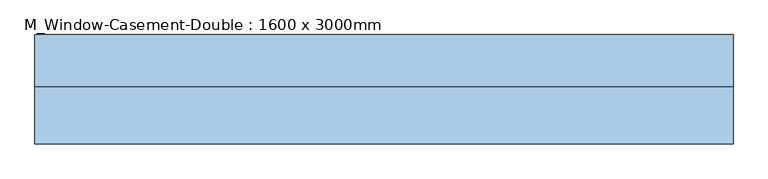
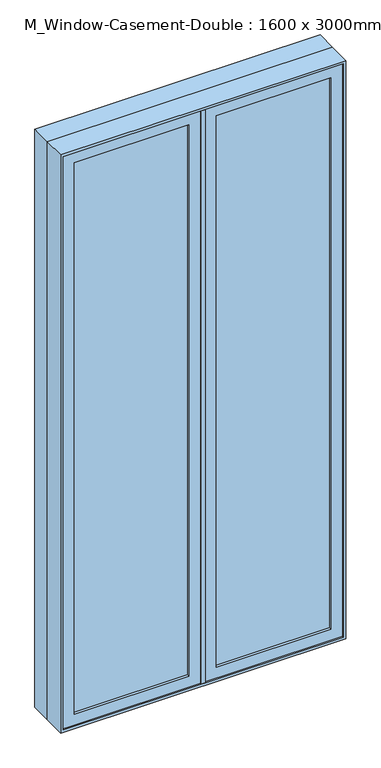
"""IFC4 building model written with IfcOpenShell, lengths in millimetres: window geometry, M_Window-Casement-Double : 1600 x 3000mm."""

import ifcopenshell
import ifcopenshell.guid

model = None  # the IFC model being written
_history = None  # IfcOwnerHistory: only IFC2X3 demands one
_inside = {}  # id of a spatial element -> (the spatial element, [elements in it])
_under = {}  # id of a project, library or spatial element -> (it, [spatial elements below it])
_declared = {}  # id of a project -> (the project, [libraries it declares])
_typed = {}  # id of a type object -> (the type object, [elements of that type])
_made_of = {}  # id of a material, layer set ... -> (it, [elements and type objects made of it])


def new_model(schema):
    """Start an empty IFC model of exactly this schema.

    Asked for "IFC4X3", IfcOpenShell would pick the latest addendum, in which some entities
    have other attributes; the version numbers below select the first issue.
    IFC2X3 requires an IfcOwnerHistory on every rooted entity: one is made here for all.
    """
    global model, _history
    if schema == "IFC4X3":
        model = ifcopenshell.file(schema_version=(4, 3, 0, 0))
    else:
        model = ifcopenshell.file(schema=schema)
    _inside.clear()
    _under.clear()
    _declared.clear()
    _typed.clear()
    _made_of.clear()
    _history = None
    if model.schema == "IFC2X3":
        org = make("IfcOrganization", Name="unknown")
        user = make(
            "IfcPersonAndOrganization",
            ThePerson=make("IfcPerson", FamilyName="unknown"),
            TheOrganization=org,
        )
        app = make(
            "IfcApplication",
            ApplicationDeveloper=org,
            Version="unknown",
            ApplicationFullName="unknown",
            ApplicationIdentifier="unknown",
        )
        _history = make(
            "IfcOwnerHistory",
            OwningUser=user,
            OwningApplication=app,
            ChangeAction="ADDED",
            CreationDate=0,
        )
    return model


def make(cls, **values):
    """One entity of the class cls with the attributes given. An attribute that is None is left unset."""
    return model.create_entity(
        cls, **{name: value for name, value in values.items() if value is not None}
    )


def rooted(cls, **values):
    """An entity with a GlobalId (a new one), such as an element, a storey or a relation."""
    return make(cls, GlobalId=ifcopenshell.guid.new(), OwnerHistory=_history, **values)


def si_unit(unit_type, name, prefix=None):
    """IfcSIUnit, for example si_unit("LENGTHUNIT", "METRE", prefix="MILLI")."""
    return make("IfcSIUnit", UnitType=unit_type, Prefix=prefix, Name=name)


def assignment(units):
    """IfcUnitAssignment: the units of a project."""
    return None if units is None else make("IfcUnitAssignment", Units=units)


def point(xyz):
    """IfcCartesianPoint."""
    return None if xyz is None else make("IfcCartesianPoint", Coordinates=xyz)


def direction(xyz):
    """IfcDirection."""
    return None if xyz is None else make("IfcDirection", DirectionRatios=xyz)


def frame(location, z_axis=None, x_axis=None):
    """IfcAxis2Placement3D, a coordinate frame: its origin and axes. An axis left out is left unset."""
    return make(
        "IfcAxis2Placement3D",
        Location=point(location),
        Axis=direction(z_axis),
        RefDirection=direction(x_axis),
    )


def origin():
    """The frame at (0, 0, 0) with its axes left unset."""
    return frame((0.0, 0.0, 0.0))


def place(relative_to, where):
    """IfcLocalPlacement: puts the frame where relative to a parent placement (None: the world)."""
    return make(
        "IfcLocalPlacement", PlacementRelTo=relative_to, RelativePlacement=where
    )


def context(
    kind, dimensions, precision=None, world=None, true_north=None, identifier=None
):
    """IfcGeometricRepresentationContext, for example the 3D "Model" context."""
    return make(
        "IfcGeometricRepresentationContext",
        ContextIdentifier=identifier,
        ContextType=kind,
        CoordinateSpaceDimension=dimensions,
        Precision=precision,
        WorldCoordinateSystem=world,
        TrueNorth=true_north,
    )


def project(units=None, contexts=None):
    """IfcProject with its units and contexts."""
    return rooted(
        "IfcProject",
        Name="project",
        RepresentationContexts=contexts,
        UnitsInContext=assignment(units),
    )


def spatial(cls, under=None, at=None, **own):
    """A site, building, storey or space (cls), placed at a placement, below another one or the project."""
    s = rooted(cls, ObjectPlacement=at, **own)
    if under is not None:
        _under.setdefault(under.id(), (under, []))[1].append(s)
    return s


def polyline(points):
    """IfcPolyline through the points."""
    return make("IfcPolyline", Points=[point(p) for p in points])


def outline(outer, holes=None, kind="AREA"):
    """IfcArbitraryClosedProfileDef: a profile drawn as a closed curve; with holes, ...WithVoids."""
    if holes is None:
        return make("IfcArbitraryClosedProfileDef", ProfileType=kind, OuterCurve=outer)
    return make(
        "IfcArbitraryProfileDefWithVoids",
        ProfileType=kind,
        OuterCurve=outer,
        InnerCurves=holes,
    )


def extrude(swept, where, along, depth):
    """IfcExtrudedAreaSolid: the profile swept, set in the frame where, extruded along a direction by depth."""
    return make(
        "IfcExtrudedAreaSolid",
        SweptArea=swept,
        Position=where,
        ExtrudedDirection=direction(along),
        Depth=depth,
    )


def faces_of(points, faces, orient=None, outer=None):
    """IfcFace entities. A face is a list of loops; a loop is a list of indices into points, from 0.

    orient and outer hold one flag for each loop. By default every Orientation is true, the
    first loop of a face is its IfcFaceOuterBound and the others are IfcFaceBound.
    """
    made = []
    for i, loops in enumerate(faces):
        bounds = []
        for j, loop in enumerate(loops):
            is_outer = j == 0 if outer is None else outer[i][j]
            bounds.append(
                make(
                    "IfcFaceOuterBound" if is_outer else "IfcFaceBound",
                    Bound=make("IfcPolyLoop", Polygon=[points[k] for k in loop]),
                    Orientation=True if orient is None else orient[i][j],
                )
            )
        made.append(make("IfcFace", Bounds=bounds))
    return made


def faceted_brep(points, faces, orient=None, outer=None, voids=None):
    """IfcFacetedBrep: a solid bounded by flat faces; with voids (closed shells), ...WithVoids."""
    shared = [point(p) for p in points]
    hull = make("IfcClosedShell", CfsFaces=faces_of(shared, faces, orient, outer))
    if voids is None:
        return make("IfcFacetedBrep", Outer=hull)
    return make(
        "IfcFacetedBrepWithVoids",
        Outer=hull,
        Voids=[
            make(cls, CfsFaces=faces_of(shared, fs, o, b)) for cls, fs, o, b in voids
        ],
    )


def shape(context_of_items, identifier, shape_type, items):
    """IfcShapeRepresentation: the items that make up one representation, for example the "Body"."""
    return make(
        "IfcShapeRepresentation",
        ContextOfItems=context_of_items,
        RepresentationIdentifier=identifier,
        RepresentationType=shape_type,
        Items=items,
    )


def source(mapping_origin, context_of_items, identifier, shape_type, items):
    """IfcRepresentationMap: a shape defined once, which mapped items show again and again."""
    return make(
        "IfcRepresentationMap",
        MappingOrigin=mapping_origin,
        MappedRepresentation=shape(context_of_items, identifier, shape_type, items),
    )


def transform(
    local_origin,
    x_axis=None,
    y_axis=None,
    z_axis=None,
    scale=None,
    scale2=None,
    scale3=None,
    uniform=True,
):
    """IfcCartesianTransformationOperator3D, or its non-uniform kind. x_axis, y_axis, z_axis: its Axis1, 2, 3."""
    if uniform:
        return make(
            "IfcCartesianTransformationOperator3D",
            Axis1=direction(x_axis),
            Axis2=direction(y_axis),
            LocalOrigin=point(local_origin),
            Scale=scale,
            Axis3=direction(z_axis),
        )
    return make(
        "IfcCartesianTransformationOperator3DnonUniform",
        Axis1=direction(x_axis),
        Axis2=direction(y_axis),
        LocalOrigin=point(local_origin),
        Scale=scale,
        Axis3=direction(z_axis),
        Scale2=scale2,
        Scale3=scale3,
    )


def mapped(mapping_source, mapping_target):
    """IfcMappedItem: shows the shape of a source again, moved by a transform."""
    return make(
        "IfcMappedItem", MappingSource=mapping_source, MappingTarget=mapping_target
    )


def made_of(thing, what):
    """Note that an element or type object is made of a material, layer set ...; save() writes the relation."""
    if what is not None:
        _made_of.setdefault(what.id(), (what, []))[1].append(thing)
    return thing


def element(
    cls,
    number,
    at=None,
    inside=None,
    cuts=None,
    type_object=None,
    material=None,
    context=None,
    identifier="Body",
    shape_type=None,
    held_by="IfcProductDefinitionShape",
    body=None,
    shapes=None,
    **own,
):
    """One element of the class cls, such as IfcWall. Its Tag is "e" and its number.

    at: its placement. inside: the storey or other place that contains it. cuts: it is an
    opening in that element (IfcRelVoidsElement). A single representation is given by context,
    identifier, shape_type and body (its items); several are given by shapes. held_by: the class
    of the entity that holds the representations. save() writes the other relations.
    """
    e = rooted(cls, Tag="e%d" % number, ObjectPlacement=at, **own)
    if body is not None:
        shapes = [shape(context, identifier, shape_type, body)]
    if shapes is not None:
        e.Representation = make(held_by, Representations=shapes)
    if inside is not None:
        _inside.setdefault(inside.id(), (inside, []))[1].append(e)
    if cuts is not None:
        rooted(
            "IfcRelVoidsElement", RelatingBuildingElement=cuts, RelatedOpeningElement=e
        )
    if type_object is not None:
        _typed.setdefault(type_object.id(), (type_object, []))[1].append(e)
    return made_of(e, material)


def aggregate(whole, parts):
    """IfcRelAggregates: a whole, such as a stair, and the parts it consists of."""
    return rooted("IfcRelAggregates", RelatingObject=whole, RelatedObjects=parts)


def save(model, path):
    """Write the relations noted so far, then the file.

    IfcRelAggregates (storeys below a building ...), IfcRelContainedInSpatialStructure (elements
    in a storey), IfcRelDefinesByType, IfcRelAssociatesMaterial and IfcRelDeclares: one each for
    every whole, place, type object, material and project.
    """
    for whole, parts in _under.values():
        aggregate(whole, parts)
    for where, things in _inside.values():
        rooted(
            "IfcRelContainedInSpatialStructure",
            RelatedElements=things,
            RelatingStructure=where,
        )
    for kind, things in _typed.values():
        rooted("IfcRelDefinesByType", RelatedObjects=things, RelatingType=kind)
    for what, things in _made_of.values():
        rooted("IfcRelAssociatesMaterial", RelatedObjects=things, RelatingMaterial=what)
    for by, libraries in _declared.values():
        rooted("IfcRelDeclares", RelatingContext=by, RelatedDefinitions=libraries)
    model.write(path)


def m_window_casement_double_1600_x_3000mm_c1f0fda9(model_context):
    return source(origin(), model_context, "Body", "SolidModel", [
        faceted_brep([(668.25, -68.25, 3868.25), (-668.25, -68.25, 3868.25), (-668.25, -4.75, 3868.25), (668.25, -4.75, 3868.25), (687.3, -119.05, 3887.3), (-687.3, -119.05, 3887.3), (-687.3, -68.25, 3887.3), (687.3, -68.25, 3887.3), (700.0, -4.75, 3900.0), (-700.0, -4.75, 3900.0), (-700.0, -119.05, 3900.0), (700.0, -119.05, 3900.0), (-668.25, -68.25, 931.75), (-668.25, -4.75, 931.75), (-687.3, -119.05, 912.7), (-687.3, -68.25, 912.7), (-700.0, -4.75, 900.0), (-700.0, -119.05, 900.0), (668.25, -68.25, 931.75), (668.25, -4.75, 931.75), (687.3, -119.05, 912.7), (687.3, -68.25, 912.7), (700.0, -4.75, 900.0), (700.0, -119.05, 900.0)], [[[0, 1, 2, 3]], [[4, 5, 6, 7]], [[8, 9, 10, 11]], [[1, 12, 13, 2]], [[5, 14, 15, 6]], [[9, 16, 17, 10]], [[12, 18, 19, 13]], [[14, 20, 21, 15]], [[16, 22, 23, 17]], [[9, 8, 22, 16], [3, 2, 13, 19]], [[18, 0, 3, 19]], [[7, 6, 15, 21], [1, 0, 18, 12]], [[20, 4, 7, 21]], [[22, 8, 11, 23]], [[11, 10, 17, 23], [5, 4, 20, 14]]]),
        extrude(outline(polyline([(3900.0, -700.0), (900.0, -700.0), (900.0, 700.0), (3900.0, 700.0), (3900.0, -700.0)]), holes=[polyline([(3880.95, 680.95), (919.05, 680.95), (919.05, -680.95), (3880.95, -680.95), (3880.95, 680.95)])]), frame((0.0, -4.75, 0.0), z_axis=(0.0, 1.0, 0.0), x_axis=(0.0, 0.0, 1.0)), (0.0, 0.0, 1.0), 104.75),
        extrude(outline(polyline([(912.7, 9.525), (912.7, 687.3), (3887.3, 687.3), (3887.3, 9.525), (912.7, 9.525)]), holes=[polyline([(969.85, 630.15), (969.85, 66.675), (3830.15, 66.675), (3830.15, 630.15), (969.85, 630.15)])]), frame((0.0, -112.7, 0.0), z_axis=(0.0, 1.0, 0.0), x_axis=(0.0, 0.0, 1.0)), (0.0, 0.0, 1.0), 44.45),
        extrude(outline(polyline([(3887.3, -9.525), (3887.3, -687.3), (912.7, -687.3), (912.7, -9.525), (3887.3, -9.525)]), holes=[polyline([(3830.15, -630.15), (3830.15, -66.675), (969.85, -66.675), (969.85, -630.15), (3830.15, -630.15)])]), frame((0.0, -112.7, 0.0), z_axis=(0.0, 1.0, 0.0), x_axis=(0.0, 0.0, 1.0)), (0.0, 0.0, 1.0), 44.45),
        extrude(outline(polyline([(630.15, -100.0), (66.675, -100.0), (66.675, -93.65), (630.15, -93.65), (630.15, -100.0)])), frame((0.0, 0.0, 969.85), z_axis=(0.0, 0.0, 1.0), x_axis=(1.0, 0.0, 0.0)), (0.0, 0.0, 1.0), 2860.3),
        extrude(outline(polyline([(66.675, -80.95), (630.15, -80.95), (630.15, -87.3), (66.675, -87.3), (66.675, -80.95)])), frame((0.0, 0.0, 969.85), z_axis=(0.0, 0.0, 1.0), x_axis=(1.0, 0.0, 0.0)), (0.0, 0.0, 1.0), 2860.3),
        extrude(outline(polyline([(-66.675, -100.0), (-630.15, -100.0), (-630.15, -93.65), (-66.675, -93.65), (-66.675, -100.0)])), frame((0.0, 0.0, 969.85), z_axis=(0.0, 0.0, 1.0), x_axis=(1.0, 0.0, 0.0)), (0.0, 0.0, 1.0), 2860.3),
        extrude(outline(polyline([(-630.15, -80.95), (-66.675, -80.95), (-66.675, -87.3), (-630.15, -87.3), (-630.15, -80.95)])), frame((0.0, 0.0, 969.85), z_axis=(0.0, 0.0, 1.0), x_axis=(1.0, 0.0, 0.0)), (0.0, 0.0, 1.0), 2860.3),
        faceted_brep([(9.525, -119.05, 3887.3), (9.525, -68.25, 3887.3), (-9.525, -68.25, 3887.3), (-9.525, -119.05, 3887.3), (9.525, -119.05, 912.7), (-9.525, -119.05, 912.7), (-9.525, -68.25, 912.7), (9.525, -68.25, 912.7), (-9.525, -68.25, 3868.25), (-9.525, -68.25, 931.75), (-30.1625, -68.25, 3868.25), (-30.1625, -68.25, 931.75), (-30.1625, -4.75, 3868.25), (-30.1625, -4.75, 931.75), (30.1625, -4.75, 3868.25), (30.1625, -4.75, 931.75), (30.1625, -68.25, 3868.25), (30.1625, -68.25, 931.75), (9.525, -68.25, 3868.25), (9.525, -68.25, 931.75)], [[[0, 1, 2, 3]], [[4, 5, 6, 7]], [[3, 5, 4, 0]], [[2, 8, 9, 6, 5, 3]], [[8, 10, 11, 9]], [[10, 12, 13, 11]], [[12, 14, 15, 13]], [[14, 16, 17, 15]], [[16, 18, 19, 17]], [[0, 4, 7, 19, 18, 1]], [[8, 2, 1, 18]], [[19, 7, 6, 9]], [[9, 11, 13, 15, 17, 19]], [[18, 16, 14, 12, 10, 8]]]),
    ])


if __name__ == "__main__":
    model = new_model("IFC4")
    model_context = context("Model", 3, world=origin())
    ifc_project = project(units=[si_unit("LENGTHUNIT", "METRE", prefix="MILLI")], contexts=[model_context])
    site = spatial("IfcSite", under=ifc_project)
    building = spatial("IfcBuilding", under=site)
    placement = place(None, origin())
    m_window_casement_double_1600_x_3000mm_shape = m_window_casement_double_1600_x_3000mm_c1f0fda9(model_context)
    element("IfcWindow", 1, ObjectType="M_Window-Casement-Double : 1600 x 3000mm", at=placement, inside=building, context=model_context, shape_type="MappedRepresentation", body=[
        mapped(m_window_casement_double_1600_x_3000mm_shape, transform((0.0, 0.0, 0.0), x_axis=(1.0, 0.0, 0.0), y_axis=(0.0, 1.0, 0.0), z_axis=(0.0, 0.0, 1.0))),
    ])
    save(model, "model.ifc")

# Revit data of these elements
# Type "M_Window-Casement-Double : 1600 x 3000mm"
#   Type Mark = "39"
#   Fire Rating = "0.5h"
#   Analytic Construction = "Double glazing - domestic"
#   Frame Extension [instance default] = 6.35 mm
#   Window Inset [instance default] = 0 mm
#   Wall Thickness [instance default] = 150 mm
#   Interior Wall Closure [instance default] = 54.75 mm
#   Half Width = 700 mm
#   Visual Light Transmittance = 0.81
#   Thermal Resistance (R) = 0.319569 (m²·K)/W
#   Solar Heat Gain Coefficient = 0.76
#   Rough Width = 1415 mm
#   Rough Height = 3015 mm
#   Height = 3000 mm
#   Heat Transfer Coefficient (U) = 3.12929 W/(m²·K)
#   Exterior Wall Closure [instance default] = 31.8 mm
#   Extension Jamb [instance default] = 54.75 mm
#   Default Sill Height = 900 mm
#   Width = 1400 mm
#   Muntin Visibility = yes
#   Interior Trim Visibility [instance default] = yes
#   Exterior Trim Visibility [instance default] = yes
#   Extension Jamb Visibility [instance default] = yes
#   Interior Trim Material = Wood - Stained
#   Muntin Pattern = M_Muntin Pattern_2x2 : M_Muntin Pattern_2x2
#   Interior Trim = M_Trim-Window-Interior-Flat : Picture Frame
#   Interior Frame Material = Wood - Stained
#   Glass Panel Material = Glass
#   Exterior Trim Material = Clad - White
#   Exterior Trim = M_Trim-Window-Exterior-Flat : with Sill
#   Exterior Frame Material = Clad - White
#   Wall Closure = (empty or 0)
# Element 1 (IfcWindow, "M_Window-Casement-Double : 1600 x 3000mm")
#   Wall Thickness = 200 mm
#   Extension Jamb = 104.75 mm
#   Materials on its faces: "Wood - Stained", "Glass", "Clad - White"
# Materials
#   "Wood - Stained": class "Wood", colour RGB 173 132 96, transparency 0, Cost = 0
#   "Glass": class "Glass", colour RGB 245 245 243, transparency 1, Description = "Soda Lime Glass", Cost = 0
#   "Clad - White": class "Wood", colour RGB 245 245 243, transparency 0, Cost = 0
